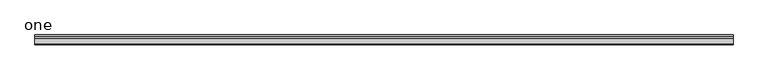
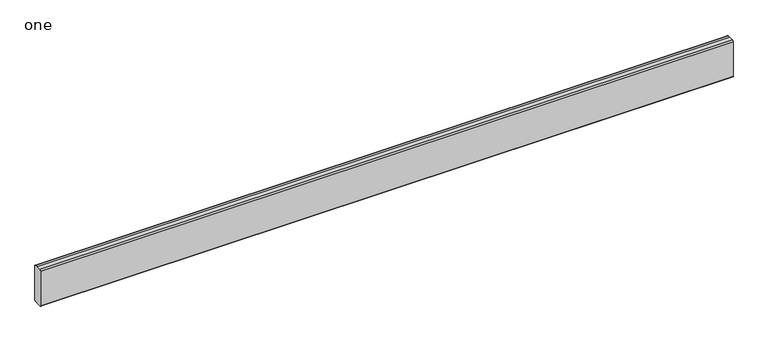
"""IFC4 building model written with IfcOpenShell, lengths in millimetres: beam geometry, Trex : one."""

from ifc_helpers import new_model, si_unit, point, frame, frame_2d, origin, place, context, project, spatial, polyline, circle_curve, trimmed, segment, composite_curve, outline, extrude, source, transform, mapped, element, save


def one_e9ea3b37(model_context):
    return source(origin(), model_context, "Body", "SweptSolid", [
        extrude(outline(composite_curve([segment(polyline([(4.9179935, -103.2371094), (-19.7941406, -103.2371094)]), True, "CONTINUOUS"), segment(trimmed(circle_curve(frame_2d((-19.7941406, -96.8871094)), 6.35), [point((-19.7941406, -103.2371094))], [point((-26.1441406, -96.8871094))], False, "CARTESIAN"), True, "CONTINUOUS"), segment(polyline([(-26.1441406, -96.8871094), (-26.1441406, 96.8871094)]), True, "CONTINUOUS"), segment(trimmed(circle_curve(frame_2d((-19.7941406, 96.8871094)), 6.35), [point((-26.1441406, 96.8871094))], [point((-19.7941406, 103.2371094))], False, "CARTESIAN"), True, "CONTINUOUS"), segment(polyline([(-19.7941406, 103.2371094), (4.9179935, 103.2371094), (4.9179935, 101.6496094), (19.7941406, 101.6496094)]), True, "CONTINUOUS"), segment(trimmed(circle_curve(frame_2d((19.7941406, 95.2996094)), 6.35), [point((19.7941406, 101.6496094))], [point((26.1441406, 95.2996094))], False, "CARTESIAN"), True, "CONTINUOUS"), segment(polyline([(26.1441406, 95.2996094), (26.1441406, -95.2996094)]), True, "CONTINUOUS"), segment(trimmed(circle_curve(frame_2d((19.7941406, -95.2996094)), 6.35), [point((26.1441406, -95.2996094))], [point((19.7941406, -101.6496094))], False, "CARTESIAN"), True, "CONTINUOUS"), segment(polyline([(19.7941406, -101.6496094), (4.9179935, -101.6496094), (4.9179935, -103.2371094)]), True, "CONTINUOUS")], self_intersect=False)), frame((-1839.0620217, 0.0, 0.0), z_axis=(1.0, 0.0, 0.0), x_axis=(0.0, 1.0, 0.0)), (0.0, 0.0, 1.0), 3678.1240435),
    ])


if __name__ == "__main__":
    model = new_model("IFC4")
    model_context = context("Model", 3, world=origin())
    ifc_project = project(units=[si_unit("LENGTHUNIT", "METRE", prefix="MILLI")], contexts=[model_context])
    site = spatial("IfcSite", under=ifc_project)
    building = spatial("IfcBuilding", under=site)
    placement = place(None, origin())
    one_shape = one_e9ea3b37(model_context)
    element("IfcBeam", 1, ObjectType="Trex : one", at=placement, inside=building, context=model_context, shape_type="MappedRepresentation", body=[
        mapped(one_shape, transform((0.0, 0.0, 0.0), x_axis=(1.0, 0.0, 0.0), y_axis=(0.0, 1.0, 0.0), z_axis=(0.0, 0.0, 1.0))),
    ])
    save(model, "model.ifc")

# Revit data of these elements
# Type "Trex : one"
#   Width = 0' - 2 15/256"
#   Web_Thickness = 0' - 0 7/64"
#   Length [instance default] = 10' - 0"
#   Leg_1 = 0' - 2 1/2"
#   Height = 0' - 8 33/256"
#   Structural Material [instance default] = none
